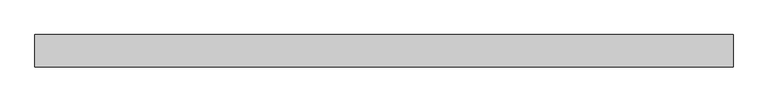
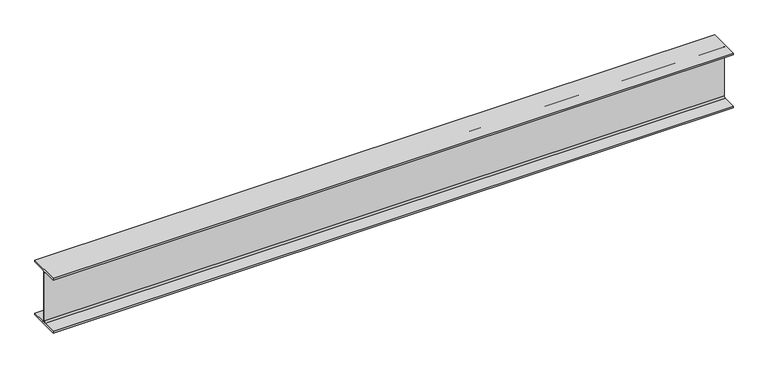
"""IFC4 building model written with IfcOpenShell, lengths in millimetres: beam geometry, Old_Steel Beam_H-KSD3502 : H_SB_ASB_H-200×200x8x12."""

from ifc_helpers import new_model, si_unit, point, frame, frame_2d, origin, place, context, project, spatial, polyline, circle_curve, trimmed, segment, composite_curve, outline, extrude, source, transform, mapped, element, save


def beam_84cdb6c9(model_context):
    return source(origin(), model_context, "Body", "SweptSolid", [
        extrude(outline(composite_curve([segment(polyline([(82.5, -141.5), (82.5, -151.7), (-82.5, -151.7), (-82.5, -141.5), (-11.9, -141.5)]), True, "CONTINUOUS"), segment(trimmed(circle_curve(frame_2d((-11.9, -132.6)), 8.9), [point((-11.9, -141.5))], [point((-3.0, -132.6))], True, "CARTESIAN"), True, "CONTINUOUS"), segment(polyline([(-3.0, -132.6), (-3.0, 132.6)]), True, "CONTINUOUS"), segment(trimmed(circle_curve(frame_2d((-11.9, 132.6)), 8.9), [point((-3.0, 132.6))], [point((-11.9, 141.5))], True, "CARTESIAN"), True, "CONTINUOUS"), segment(polyline([(-11.9, 141.5), (-82.5, 141.5), (-82.5, 151.7), (82.5, 151.7), (82.5, 141.5), (11.9, 141.5)]), True, "CONTINUOUS"), segment(trimmed(circle_curve(frame_2d((11.9, 132.6)), 8.9), [point((11.9, 141.5))], [point((3.0, 132.6))], True, "CARTESIAN"), True, "CONTINUOUS"), segment(polyline([(3.0, 132.6), (3.0, -132.6)]), True, "CONTINUOUS"), segment(trimmed(circle_curve(frame_2d((11.9, -132.6)), 8.9), [point((3.0, -132.6))], [point((11.9, -141.5))], True, "CARTESIAN"), True, "CONTINUOUS"), segment(polyline([(11.9, -141.5), (82.5, -141.5)]), True, "CONTINUOUS")], self_intersect=False)), frame((-1734.3504002, 0.0, 0.0), z_axis=(1.0, 0.0, 0.0), x_axis=(0.0, 1.0, 0.0)), (0.0, 0.0, 1.0), 3554.555596),
    ])


if __name__ == "__main__":
    model = new_model("IFC4")
    model_context = context("Model", 3, world=origin())
    ifc_project = project(units=[si_unit("LENGTHUNIT", "METRE", prefix="MILLI")], contexts=[model_context])
    site = spatial("IfcSite", under=ifc_project)
    building = spatial("IfcBuilding", under=site)
    placement = place(None, origin())
    beam_shape = beam_84cdb6c9(model_context)
    element("IfcBeam", 1, ObjectType="Old_Steel Beam_H-KSD3502 : H_SB_ASB_H-200×200x8x12", at=placement, inside=building, context=model_context, shape_type="MappedRepresentation", body=[
        mapped(beam_shape, transform((0.0, 0.0, 0.0), x_axis=(1.0, 0.0, 0.0), y_axis=(0.0, 1.0, 0.0), z_axis=(0.0, 0.0, 1.0))),
    ])
    save(model, "model.ifc")

# Revit data of these elements
# Type "Old_Steel Beam_H-KSD3502 : H_SB_ASB_H-200×200x8x12"
#   Width = 20.0 cm
#   Web Thickness = 0.8 cm
#   Web Fillet = 1.3 cm
#   Warping Constant = 141376.0 cm⁶
#   Torsional Moment of Inertia = 26.2485 cm⁴
#   Torsional Modulus = 1.0 cm³
#   Section Area = 63.53 cm²
#   Plastic Modulus weak axis = 244.0 cm³
#   Plastic Modulus strong axis = 525.0 cm³
#   Perimeter = 1.16 m²/m
#   Nominal Weight = 49.90 kgf/m
#   Moment of Inertia weak axis = 1600.00 cm⁴
#   Moment of Inertia strong axis = 4720.00 cm⁴
#   Height = 20.0 cm
#   Flange Thickness = 1.2 cm
#   Elastic Modulus weak axis = 160.0 cm³
#   Elastic Modulus strong axis = 472.0 cm³
#   Centroid Vertical = 10.0 cm
#   Centroid Horizontal = 10.0 cm
#   Length [instance default] = 1.5240 m
#   Structural Material [instance default] = Steel, 45-345
#   Assembly Code = ""
# Element 1 (IfcBeam, "Old_Steel Beam_H-KSD3502 : H_SB_ASB_H-200×200x8x12")
#   Structural Material = none
# Materials
#   "Steel, 45-345": class "Metal", colour RGB 189 187 185, transparency 0, Description = "Steel 345 MPa", Cost = 0
